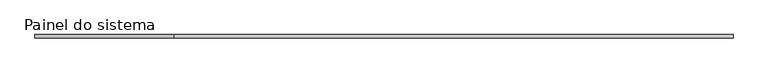
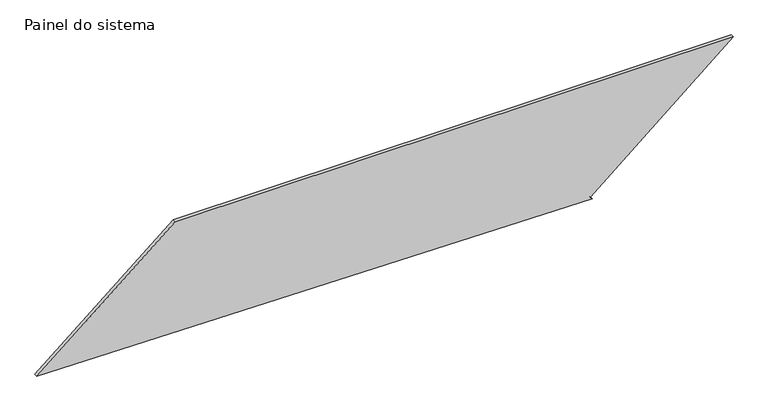
"""IFC4 building model written with IfcOpenShell, lengths in millimetres: plate geometry, Painel do sistema : Envidraçado."""

from ifc_helpers import new_model, si_unit, frame, origin, place, context, project, spatial, polyline, outline, extrude, source, transform, mapped, element, save


def painel_do_sistema_2fe3f8c8(model_context):
    return source(origin(), model_context, "Body", "SweptSolid", [
        extrude(outline(polyline([(0.0, 1478.5677973), (19.2037959, 1462.5611042), (869.2425761, 2482.3826979), (869.2425761, -1496.6230553), (47.595016, -2482.3826979), (0.0, 1478.5677973)])), frame((0.0, 24.5, 0.0), z_axis=(0.0, 1.0, 0.0), x_axis=(0.0, 0.0, 1.0)), (0.0, 0.0, 1.0), 25.0),
    ])


if __name__ == "__main__":
    model = new_model("IFC4")
    model_context = context("Model", 3, world=origin())
    ifc_project = project(units=[si_unit("LENGTHUNIT", "METRE", prefix="MILLI")], contexts=[model_context])
    site = spatial("IfcSite", under=ifc_project)
    building = spatial("IfcBuilding", under=site)
    placement = place(None, origin())
    painel_do_sistema_shape = painel_do_sistema_2fe3f8c8(model_context)
    element("IfcPlate", 1, ObjectType="Painel do sistema : Envidraçado", at=placement, inside=building, context=model_context, shape_type="MappedRepresentation", body=[
        mapped(painel_do_sistema_shape, transform((0.0, 0.0, 0.0), x_axis=(1.0, 0.0, 0.0), y_axis=(0.0, 1.0, 0.0), z_axis=(0.0, 0.0, 1.0))),
    ])
    save(model, "model.ifc")

# Revit data of these elements
# Type "Painel do sistema : Envidraçado"
#   Construction Type Id = "GSP4R"
#   Analytic Construction = "Vidraça única Pilkington 1/8 pol"
#   Visual Light Transmittance = 0.9
#   Solar Heat Gain Coefficient = 0.86
#   Heat Transfer Coefficient (U) = 6.7069 W/(m²·K)
# Element 1 (IfcPlate, "Painel do sistema : Envidraçado")
#   Materials on its faces: "Vidro"
# Materials
#   "Vidro": class "Vidro", colour RGB 0 128 192, transparency 0.9, Description = "Vidro de sílica", Cost = 0
